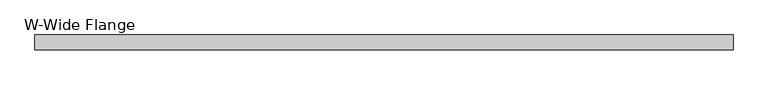
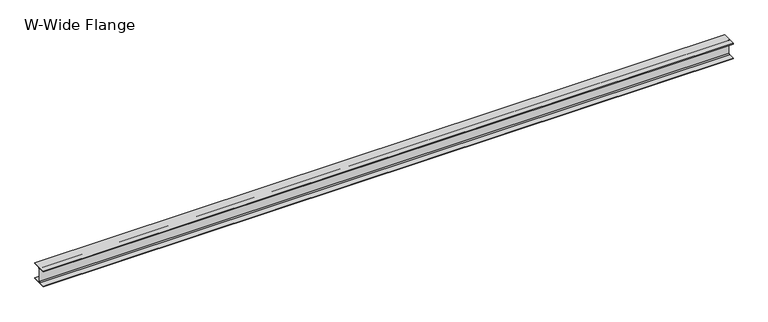
"""IFC4 building model written with IfcOpenShell, lengths in millimetres: beam geometry, W-Wide Flange."""

from ifc_helpers import new_model, si_unit, point, frame, frame_2d, origin, place, context, project, spatial, polyline, circle_curve, trimmed, segment, composite_curve, outline, extrude, source, transform, mapped, element, save


def w_wide_flange_e536b83e(model_context):
    return source(origin(), model_context, "Body", "SweptSolid", [
        extrude(outline(composite_curve([segment(polyline([(95.25, -97.2185), (95.25, -106.3625), (-95.25, -106.3625), (-95.25, -97.2185), (-17.7165, -97.2185)]), True, "CONTINUOUS"), segment(trimmed(circle_curve(frame_2d((-17.7165, -82.55)), 14.6685), [point((-17.7165, -97.2185))], [point((-3.048, -82.55))], True, "CARTESIAN"), True, "CONTINUOUS"), segment(polyline([(-3.048, -82.55), (-3.048, 82.55)]), True, "CONTINUOUS"), segment(trimmed(circle_curve(frame_2d((-17.7165, 82.55)), 14.6685), [point((-3.048, 82.55))], [point((-17.7165, 97.2185))], True, "CARTESIAN"), True, "CONTINUOUS"), segment(polyline([(-17.7165, 97.2185), (-95.25, 97.2185), (-95.25, 106.3625), (95.25, 106.3625), (95.25, 97.2185), (17.7165, 97.2185)]), True, "CONTINUOUS"), segment(trimmed(circle_curve(frame_2d((17.7165, 82.55)), 14.6685), [point((17.7165, 97.2185))], [point((3.048, 82.55))], True, "CARTESIAN"), True, "CONTINUOUS"), segment(polyline([(3.048, 82.55), (3.048, -82.55)]), True, "CONTINUOUS"), segment(trimmed(circle_curve(frame_2d((17.7165, -82.55)), 14.6685), [point((3.048, -82.55))], [point((17.7165, -97.2185))], True, "CARTESIAN"), True, "CONTINUOUS"), segment(polyline([(17.7165, -97.2185), (95.25, -97.2185)]), True, "CONTINUOUS")], self_intersect=False)), frame((-4445.1356486, 0.0, 0.0), z_axis=(1.0, 0.0, 0.0), x_axis=(0.0, 1.0, 0.0)), (0.0, 0.0, 1.0), 8890.2712971),
    ])


if __name__ == "__main__":
    model = new_model("IFC4")
    model_context = context("Model", 3, world=origin())
    ifc_project = project(units=[si_unit("LENGTHUNIT", "METRE", prefix="MILLI")], contexts=[model_context])
    site = spatial("IfcSite", under=ifc_project)
    building = spatial("IfcBuilding", under=site)
    placement = place(None, origin())
    w_wide_flange_shape = w_wide_flange_e536b83e(model_context)
    element("IfcBeam", 1, ObjectType="W-Wide Flange : ODD SIZE (8 3/8\" D x 7 1/2\" W)", at=placement, inside=building, context=model_context, shape_type="MappedRepresentation", body=[
        mapped(w_wide_flange_shape, transform((0.0, 0.0, 0.0), x_axis=(1.0, 0.0, 0.0), y_axis=(0.0, 1.0, 0.0), z_axis=(0.0, 0.0, 1.0))),
    ])
    save(model, "model.ifc")

# Revit data of these elements
# Type "W-Wide Flange : ODD SIZE (8 3/8\" D x 7 1/2\" W)"
#   Assembly Code = "B10"
#   W = 22
#   Length [instance default] = 5' - 0"
#   bf = 0' - 7 1/2"
#   d = 0' - 8 3/8"
#   k = 0' - 0 15/16"
#   k2 = 0' - 0.5775"
#   tf = 0' - 0.36"
#   tw = 0' - 0.24"
#   A = 0.0450694 SF
#   Structural Material [instance default] = Steel ASTM A992
# Element 1 (IfcBeam, "W-Wide Flange : ODD SIZE (8 3/8\" D x 7 1/2\" W)")
#   Materials on its faces: "Steel ASTM A992"
# Materials
#   "Steel ASTM A992": class "Metal", colour RGB 199 199 199, transparency 0, Description = "Structural steel 50ksi", Cost = 0
